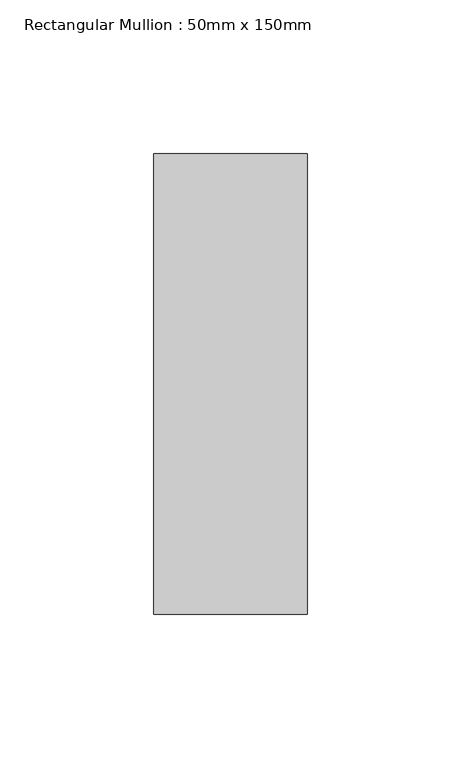
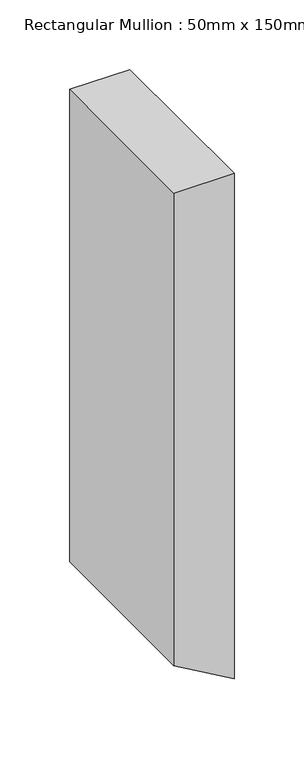
"""IFC4 building model written with IfcOpenShell, lengths in millimetres: member geometry, Rectangular Mullion : 50mm x 150mm."""

from ifc_helpers import new_model, si_unit, frame, origin, place, context, project, spatial, polyline, outline, extrude, source, transform, mapped, element, save


def rectangular_mullion_50mm_x_150mm_8d818d6c(model_context):
    return source(origin(), model_context, "Body", "SweptSolid", [
        extrude(outline(polyline([(0.0, 25.0), (0.0, -25.0), (-414.6250782, -25.0), (-443.4925917, 25.0), (0.0, 25.0)])), frame((0.0, -75.0, 0.0), z_axis=(0.0, 1.0, 0.0), x_axis=(0.0, 0.0, 1.0)), (0.0, 0.0, 1.0), 150.0),
    ])


if __name__ == "__main__":
    model = new_model("IFC4")
    model_context = context("Model", 3, world=origin())
    ifc_project = project(units=[si_unit("LENGTHUNIT", "METRE", prefix="MILLI")], contexts=[model_context])
    site = spatial("IfcSite", under=ifc_project)
    building = spatial("IfcBuilding", under=site)
    placement = place(None, origin())
    rectangular_mullion_50mm_x_150mm_shape = rectangular_mullion_50mm_x_150mm_8d818d6c(model_context)
    element("IfcMember", 1, ObjectType="Rectangular Mullion : 50mm x 150mm", at=placement, inside=building, context=model_context, shape_type="MappedRepresentation", body=[
        mapped(rectangular_mullion_50mm_x_150mm_shape, transform((0.0, 0.0, 0.0), x_axis=(1.0, 0.0, 0.0), y_axis=(0.0, 1.0, 0.0), z_axis=(0.0, 0.0, 1.0))),
    ])
    save(model, "model.ifc")

# Revit data of these elements
# Type "Rectangular Mullion : 50mm x 150mm"
#   built-in parameter 1007304 = 0.492126 (stored number, unit not read)
#   built-in parameter 1007301 = 0.082021 (stored number, unit not read)
#   built-in parameter 1007300 = 0.082021 (stored number, unit not read)
# Element 1 (IfcMember, "Rectangular Mullion : 50mm x 150mm")
#   Materials on its faces: "Aluminum"
# Materials
#   "Aluminum": class "Metal", colour RGB 247 247 247, transparency 0, Description = "Aluminum 6061", Cost = 0
